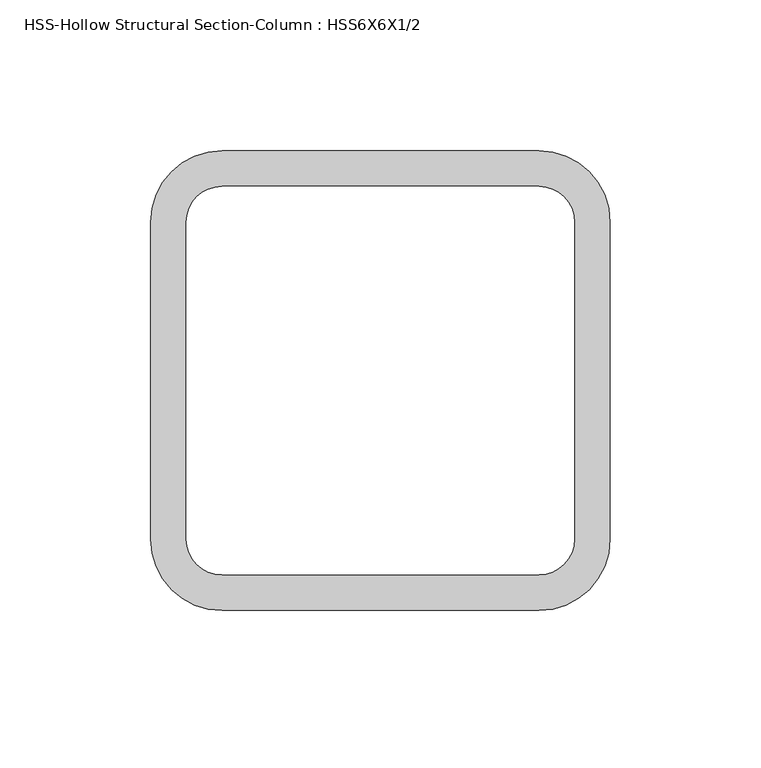
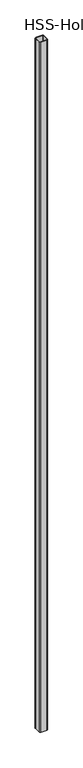
"""IFC4 building model written with IfcOpenShell, lengths in millimetres: column geometry, HSS-Hollow Structural Section-Column : HSS6X6X1/2."""

from ifc_helpers import new_model, si_unit, point, frame, frame_2d, origin, place, context, project, spatial, polyline, circle_curve, trimmed, segment, composite_curve, outline, extrude, source, transform, mapped, element, save


def hss_hollow_structural_section_column_hss6x6x1_2_34949b0c(model_context):
    return source(origin(), model_context, "Body", "SweptSolid", [
        extrude(outline(composite_curve([segment(trimmed(circle_curve(frame_2d((52.578, 52.578)), 23.622), [point((52.578, 76.2))], [point((76.2, 52.578))], False, "CARTESIAN"), True, "CONTINUOUS"), segment(polyline([(76.2, 52.578), (76.2, -52.578)]), True, "CONTINUOUS"), segment(trimmed(circle_curve(frame_2d((52.578, -52.578)), 23.622), [point((76.2, -52.578))], [point((52.578, -76.2))], False, "CARTESIAN"), True, "CONTINUOUS"), segment(polyline([(52.578, -76.2), (-52.578, -76.2)]), True, "CONTINUOUS"), segment(trimmed(circle_curve(frame_2d((-52.578, -52.578)), 23.622), [point((-52.578, -76.2))], [point((-76.2, -52.578))], False, "CARTESIAN"), True, "CONTINUOUS"), segment(polyline([(-76.2, -52.578), (-76.2, 52.578)]), True, "CONTINUOUS"), segment(trimmed(circle_curve(frame_2d((-52.578, 52.578)), 23.622), [point((-76.2, 52.578))], [point((-52.578, 76.2))], False, "CARTESIAN"), True, "CONTINUOUS"), segment(polyline([(-52.578, 76.2), (52.578, 76.2)]), True, "CONTINUOUS")], self_intersect=False), holes=[composite_curve([segment(polyline([(52.578, 64.389), (-52.578, 64.389)]), True, "CONTINUOUS"), segment(trimmed(circle_curve(frame_2d((-52.578, 52.578)), 11.811), [point((-52.578, 64.389))], [point((-64.389, 52.578))], True, "CARTESIAN"), True, "CONTINUOUS"), segment(polyline([(-64.389, 52.578), (-64.389, -52.578)]), True, "CONTINUOUS"), segment(trimmed(circle_curve(frame_2d((-52.578, -52.578)), 11.811), [point((-64.389, -52.578))], [point((-52.578, -64.389))], True, "CARTESIAN"), True, "CONTINUOUS"), segment(polyline([(-52.578, -64.389), (52.578, -64.389)]), True, "CONTINUOUS"), segment(trimmed(circle_curve(frame_2d((52.578, -52.578)), 11.811), [point((52.578, -64.389))], [point((64.389, -52.578))], True, "CARTESIAN"), True, "CONTINUOUS"), segment(polyline([(64.389, -52.578), (64.389, 52.578)]), True, "CONTINUOUS"), segment(trimmed(circle_curve(frame_2d((52.578, 52.578)), 11.811), [point((64.389, 52.578))], [point((52.578, 64.389))], True, "CARTESIAN"), True, "CONTINUOUS")], self_intersect=False)]), frame((0.0, 0.0, -609.6), z_axis=(0.0, 0.0, 1.0), x_axis=(1.0, 0.0, 0.0)), (0.0, 0.0, 1.0), 12877.8),
    ])


if __name__ == "__main__":
    model = new_model("IFC4")
    model_context = context("Model", 3, world=origin())
    ifc_project = project(units=[si_unit("LENGTHUNIT", "METRE", prefix="MILLI")], contexts=[model_context])
    site = spatial("IfcSite", under=ifc_project)
    building = spatial("IfcBuilding", under=site)
    placement = place(None, origin())
    hss_hollow_structural_section_column_hss6x6x1_2_shape = hss_hollow_structural_section_column_hss6x6x1_2_34949b0c(model_context)
    element("IfcColumn", 1, ObjectType="HSS-Hollow Structural Section-Column : HSS6X6X1/2", at=placement, inside=building, context=model_context, shape_type="MappedRepresentation", body=[
        mapped(hss_hollow_structural_section_column_hss6x6x1_2_shape, transform((0.0, 0.0, 0.0), x_axis=(1.0, 0.0, 0.0), y_axis=(0.0, 1.0, 0.0), z_axis=(0.0, 0.0, 1.0))),
    ])
    save(model, "model.ifc")

# Revit data of these elements
# Type "HSS-Hollow Structural Section-Column : HSS6X6X1/2"
#   Assembly Code = "B10"
#   Shape = "Square"
#   W = 35.1
#   Ht = 0' - 6"
#   b = 0' - 6"
#   kr = 0' - 0.93"
#   t = 0' - 0.465"
#   A = 0.0676389 SF
#   Structural Material [instance default] = Steel ASTM A500, Grade B, Rectangular and Square
# Element 1 (IfcColumn, "HSS-Hollow Structural Section-Column : HSS6X6X1/2")
#   Materials on its faces: "Steel ASTM A500, Grade B, Rectangular and Square"
# Materials
#   "Steel ASTM A500, Grade B, Rectangular and Square": class "Metal", colour RGB 199 199 199, transparency 0, Description = "Carbon steel", Cost = 0
